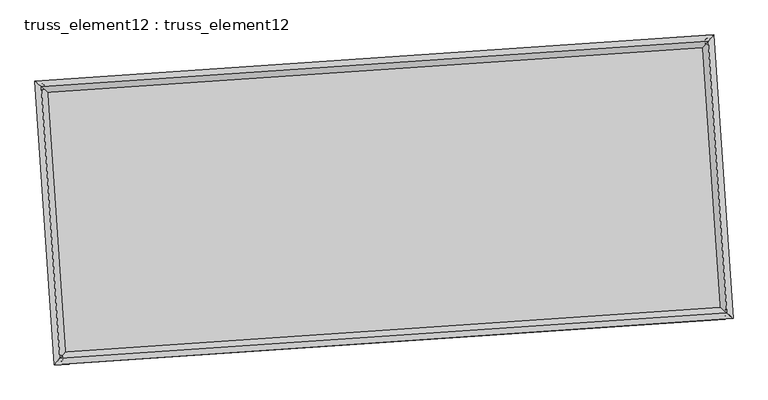
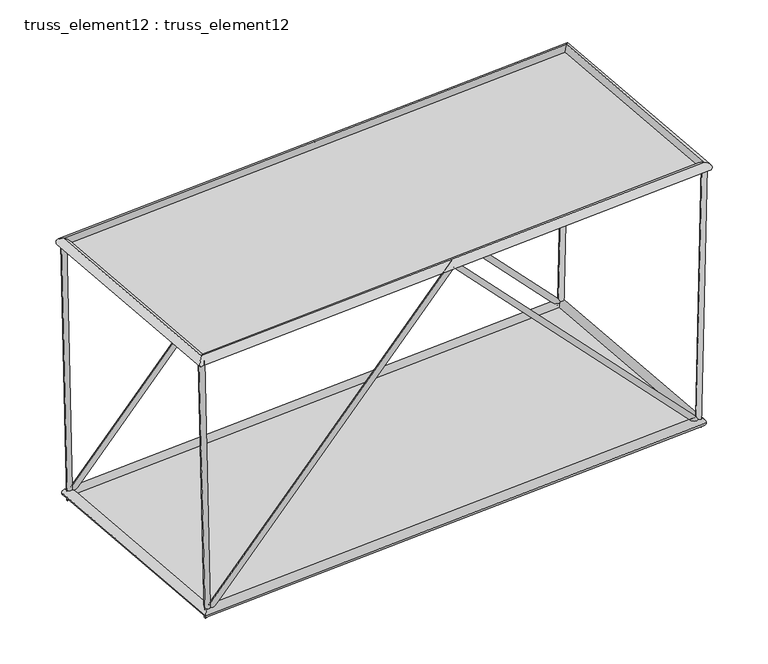
"""IFC4 building model written with IfcOpenShell, lengths in millimetres: plate geometry, truss_element12 : truss_element12."""

from ifc_helpers import new_model, si_unit, frame, origin, origin_with_axes, place, context, project, spatial, polyline, circle_curve, ellipse_curve, outline, extrude, source, transform, mapped, element, save
from ifc_brep_helpers import plane_surface, cylinder_surface, advanced_brep


def truss_element12_truss_element12_67497611(model_context):
    return source(origin(), model_context, "Body", "SolidModel", [
        advanced_brep(
        [(-3780.0029649, 2268.3783734, 4999.8207113), (-3879.0798521, 2255.0189396, 4997.5194202), (-3667.7199382, 2276.0345262, 121.2833616), (-3761.2669446, 2263.0521539, -121.2833616), (1063.4080842, 2598.6321613, 5070.7911986), (1063.8609339, 2592.0592819, 4926.563185), (5795.1440194, 2921.2712477, 121.2875843), (5889.6169576, 2921.1092408, -121.2875843), (5906.8236398, 2928.8862565, 4999.8287822), (6006.7972134, 2929.099317, 4997.5398535)],
        [
            (0, 1, circle_curve(frame((-3829.5414085, 2261.6986565, 4998.6700657), z_axis=(-0.023009593417978043, -0.0015689367075187464, 0.9997340131496714), x_axis=(-0.13359490987077044, 0.9910348587124408, -0.0015194977569957108)), 50.0)),
            (1, 0, circle_curve(frame((-3829.5414085, 2261.6986565, 4998.6700657), z_axis=(-0.023009593417978043, -0.0015689367075187464, 0.9997340131496714), x_axis=(-0.13359490987077044, 0.9910348587124408, -0.0015194977569957108)), 50.0)),
            (0, 2),
            (2, 3, ellipse_curve(frame((-3714.4934414, 2269.54334, 0.0), z_axis=(-0.9299983802713419, -0.06341305429589184, 0.36205220236527585), x_axis=(0.36121347081217686, 0.024629773473731183, 0.9321578207376976)), 130.3936428, 50.0)),
            (3, 1),
            (3, 2, ellipse_curve(frame((-3714.4934414, 2269.54334, 0.0), z_axis=(-0.9299983802713419, -0.06341305429589184, 0.36205220236527585), x_axis=(0.36121347081217686, 0.024629773473731183, 0.9321578207376976)), 130.3936428, 50.0)),
            (2, 4),
            (4, 5, ellipse_curve(frame((1063.6345091, 2595.3457216, 4998.6771918), z_axis=(-0.9976833955542868, -0.06802823819320505, -3.230475386094174e-05), x_axis=(3.22299165412689e-05, 2.1976354916597875e-06, -0.9999999994782015)), 72.2710337, 50.0)),
            (5, 3),
            (5, 4, ellipse_curve(frame((1063.6345091, 2595.3457216, 4998.6771918), z_axis=(-0.9976833955542868, -0.06802823819320505, -3.230475386094174e-05), x_axis=(3.22299165412689e-05, 2.1976354916597875e-06, -0.9999999994782015)), 72.2710337, 50.0)),
            (4, 6),
            (6, 7, ellipse_curve(frame((5842.3804885, 2921.1902443, 0.0), z_axis=(-0.9299643254301767, -0.0634107322257276, -0.36214007299081596), x_axis=(-0.3613011378762809, -0.02463575115757878, 0.9321236868217686)), 130.4029578, 50.0)),
            (7, 5),
            (7, 6, ellipse_curve(frame((5842.3804885, 2921.1902443, 0.0), z_axis=(-0.9299643254301767, -0.0634107322257276, -0.36214007299081596), x_axis=(-0.3613011378762809, -0.02463575115757878, 0.9321236868217686)), 130.4029578, 50.0)),
            (8, 9, circle_curve(frame((5956.8104266, 2928.9927867, 4998.6843179), z_axis=(0.02288598762129972, 0.001560508498112905, 0.9997368635715226), x_axis=(-0.002165762489590564, 0.9999965126634012, -0.0015113351298953748)), 50.0)),
            (9, 8, circle_curve(frame((5956.8104266, 2928.9927867, 4998.6843179), z_axis=(0.02288598762129972, 0.001560508498112905, 0.9997368635715226), x_axis=(-0.002165762489590564, 0.9999965126634012, -0.0015113351298953748)), 50.0)),
            (6, 8),
            (9, 7),
        ],
        [
            plane_surface(frame((-3829.5414085, 2311.6985949, 4998.7485334), z_axis=(-0.023009593417979597, -0.0015689367075153488, 0.9997340131496715), x_axis=(0.9997352442575682, -3.611015610971435e-05, 0.023009565083185635))),
            cylinder_surface(frame((-3829.5414085, 2261.6986565, 4998.6700657), z_axis=(-0.023009593417978046, -0.0015689367075187469, 0.9997340131496716), x_axis=(-0.13359490987077044, 0.9910348587124408, -0.0015194977569957108)), 50.0),
            cylinder_surface(frame((-3714.4934414, 2269.54334, 0.0), z_axis=(-0.6902141194664027, -0.04706307705691265, -0.7220730822203205), x_axis=(-0.02041714812690732, 0.9987520200568047, -0.04558006685839855)), 50.0),
            cylinder_surface(frame((1063.6345091, 2595.3457216, 4998.6771918), z_axis=(-0.6902606627361209, -0.04706625066554735, 0.722028382771328), x_axis=(-0.11534077341471446, 0.9922795388869102, -0.045583140463075246)), 50.0),
            plane_surface(frame((5956.8104266, 2878.9928477, 4998.7623637), z_axis=(0.022885987621301448, 0.0015605084981140682, 0.9997368635715226), x_axis=(0.9997380814846446, -3.572313472055558e-05, -0.02288595974085441))),
            cylinder_surface(frame((5842.3804885, 2921.1902443, 0.0), z_axis=(-0.02288598762129972, -0.001560508498112905, -0.9997368635715226), x_axis=(-0.002165762489590564, 0.9999965126634012, -0.0015113351298953748)), 50.0),
        ],
        [
            (0, [[1, 2]]),
            (1, [[-1, 3, 4, 5]]),
            (1, [[-2, -5, 6, -3]]),
            (2, [[-4, 7, 8, 9]]),
            (2, [[-6, -9, 10, -7]]),
            (3, [[-8, 11, 12, 13]]),
            (3, [[-10, -13, 14, -11]]),
            (4, [[15, 16]]),
            (5, [[-12, 17, -16, 18]]),
            (5, [[-14, -18, -15, -17]]),
        ],
    ),
        advanced_brep(
        [(-3507.890012, -1722.3552109, 4999.8207113), (-3606.9668992, -1735.7146447, 4997.5194202), (-3395.6069853, -1714.6990581, 121.2833616), (-3489.1539917, -1727.6814304, -121.2833616), (1335.5210371, -1392.101423, 5070.7911986), (1335.9738868, -1398.6743024, 4926.563185), (6067.2569723, -1069.4623366, 121.2875843), (6161.7299105, -1069.6243435, -121.2875843), (6178.9365927, -1061.8473278, 4999.8287822), (6278.9101663, -1061.6342673, 4997.5398535)],
        [
            (0, 1, circle_curve(frame((-3557.4284556, -1729.0349278, 4998.6700657), z_axis=(-0.02300959341797794, -0.0015689367075187003, 0.9997340131496715), x_axis=(-0.13359490987077055, 0.9910348587124407, -0.0015194977569957455)), 50.0)),
            (1, 0, circle_curve(frame((-3557.4284556, -1729.0349278, 4998.6700657), z_axis=(-0.02300959341797794, -0.0015689367075187003, 0.9997340131496715), x_axis=(-0.13359490987077055, 0.9910348587124407, -0.0015194977569957455)), 50.0)),
            (0, 2),
            (2, 3, ellipse_curve(frame((-3442.3804885, -1721.1902443, 0.0), z_axis=(-0.9299983802713419, -0.0634130542958918, 0.3620522023652762), x_axis=(0.3612134708121772, 0.02462977347373123, 0.9321578207376975)), 130.3936428, 50.0)),
            (3, 1),
            (3, 2, ellipse_curve(frame((-3442.3804885, -1721.1902443, 0.0), z_axis=(-0.9299983802713419, -0.0634130542958918, 0.3620522023652762), x_axis=(0.3612134708121772, 0.02462977347373123, 0.9321578207376975)), 130.3936428, 50.0)),
            (2, 4),
            (4, 5, ellipse_curve(frame((1335.747462, -1395.3878627, 4998.6771918), z_axis=(-0.9976833955542868, -0.06802823819320494, -3.230475386070103e-05), x_axis=(3.222991654111514e-05, 2.1976354915444677e-06, -0.9999999994782015)), 72.2710337, 50.0)),
            (5, 3),
            (5, 4, ellipse_curve(frame((1335.747462, -1395.3878627, 4998.6771918), z_axis=(-0.9976833955542868, -0.06802823819320494, -3.230475386070103e-05), x_axis=(3.222991654111514e-05, 2.1976354915444677e-06, -0.9999999994782015)), 72.2710337, 50.0)),
            (4, 6),
            (6, 7, ellipse_curve(frame((6114.4934414, -1069.54334, 0.0), z_axis=(-0.9299643254301767, -0.0634107322257272, -0.36214007299081574), x_axis=(-0.3613011378762808, -0.02463575115757876, 0.9321236868217685)), 130.4029578, 50.0)),
            (7, 5),
            (7, 6, ellipse_curve(frame((6114.4934414, -1069.54334, 0.0), z_axis=(-0.9299643254301767, -0.0634107322257272, -0.36214007299081574), x_axis=(-0.3613011378762808, -0.02463575115757876, 0.9321236868217685)), 130.4029578, 50.0)),
            (8, 9, circle_curve(frame((6228.9233795, -1061.7407976, 4998.6843179), z_axis=(0.02288598762129982, 0.0015605084981127825, 0.9997368635715226), x_axis=(-0.002165762489590051, 0.9999965126634012, -0.001511335129895264)), 50.0)),
            (9, 8, circle_curve(frame((6228.9233795, -1061.7407976, 4998.6843179), z_axis=(0.02288598762129982, 0.0015605084981127825, 0.9997368635715226), x_axis=(-0.002165762489590051, 0.9999965126634012, -0.001511335129895264)), 50.0)),
            (6, 8),
            (9, 7),
        ],
        [
            plane_surface(frame((-3557.4284556, -1679.0349894, 4998.7485334), z_axis=(-0.023009593417979597, -0.0015689367075153446, 0.9997340131496715), x_axis=(0.9997352442575682, -3.611015610971435e-05, 0.023009565083185635))),
            cylinder_surface(frame((-3557.4284556, -1729.0349278, 4998.6700657), z_axis=(-0.023009593417977935, -0.0015689367075186998, 0.9997340131496713), x_axis=(-0.13359490987077055, 0.9910348587124407, -0.0015194977569957455)), 50.0),
            cylinder_surface(frame((-3442.3804885, -1721.1902443, 0.0), z_axis=(-0.6902141194664028, -0.04706307705691266, -0.7220730822203204), x_axis=(-0.0204171481269073, 0.9987520200568046, -0.04558006685839858)), 50.0),
            cylinder_surface(frame((1335.747462, -1395.3878627, 4998.6771918), z_axis=(-0.6902606627361206, -0.04706625066554716, 0.7220283827713282), x_axis=(-0.11534077341471438, 0.9922795388869101, -0.04558314046307537)), 50.0),
            plane_surface(frame((6228.9233795, -1111.7407366, 4998.7623637), z_axis=(0.022885987621301448, 0.001560508498114064, 0.9997368635715226), x_axis=(0.9997380814846446, -3.572313472099967e-05, -0.02288595974085441))),
            cylinder_surface(frame((6114.4934414, -1069.54334, 0.0), z_axis=(-0.02288598762129982, -0.0015605084981127825, -0.9997368635715226), x_axis=(-0.002165762489590051, 0.9999965126634012, -0.001511335129895264)), 50.0),
        ],
        [
            (0, [[1, 2]]),
            (1, [[-1, 3, 4, 5]]),
            (1, [[-2, -5, 6, -3]]),
            (2, [[-4, 7, 8, 9]]),
            (2, [[-6, -9, 10, -7]]),
            (3, [[-8, 11, 12, 13]]),
            (3, [[-10, -13, 14, -11]]),
            (4, [[15, 16]]),
            (5, [[-12, 17, -16, 18]]),
            (5, [[-14, -18, -15, -17]]),
        ],
    ),
        advanced_brep(
        [(-3557.4247553, -1729.0308266, 4908.6700658), (-3557.4321559, -1729.039029, 5088.6700657), (-3829.5456313, 2261.7022175, 5088.6700657), (-3829.5371857, 2261.6950955, 4908.6700658), (5956.813866, 2928.9968702, 5088.6843178), (5956.8069872, 2928.9887033, 4908.6843179), (6228.9273414, -1061.7443763, 5088.6843178), (6228.9194177, -1061.7372188, 4908.6843179)],
        [
            (0, 1, ellipse_curve(frame((-3557.4284556, -1729.0349278, 4998.6700657), z_axis=(-0.7535719234047118, 0.6573654662781334, -1.0273917259752128e-06), x_axis=(-0.657365466277338, -0.7535719234054056, -1.0273917259753225e-06)), 127.2792206, 90.0)),
            (1, 2),
            (2, 3, ellipse_curve(frame((-3829.5414085, 2261.6986565, 4998.6700657), z_axis=(-0.657365466277338, -0.7535719234054056, -1.027391725975426e-06), x_axis=(0.7535719234047117, -0.6573654662781334, 1.0273917259753161e-06)), 127.2792206, 90.0)),
            (3, 0),
            (1, 0, ellipse_curve(frame((-3557.4284556, -1729.0349278, 4998.6700657), z_axis=(-0.7535719234047118, 0.6573654662781334, -1.0273917259752128e-06), x_axis=(-0.657365466277338, -0.7535719234054056, -1.0273917259753225e-06)), 127.2792206, 90.0)),
            (3, 2, ellipse_curve(frame((-3829.5414085, 2261.6986565, 4998.6700657), z_axis=(-0.657365466277338, -0.7535719234054056, -1.027391725975426e-06), x_axis=(0.7535719234047117, -0.6573654662781334, 1.0273917259753161e-06)), 127.2792206, 90.0)),
            (2, 4),
            (4, 5, ellipse_curve(frame((5956.8104266, 2928.9927867, 4998.6843179), z_axis=(-0.7535719234047119, 0.6573654662781332, -1.027391725975419e-06), x_axis=(-0.6573654662773378, -0.7535719234054058, -1.0273917259753231e-06)), 127.2792206, 90.0)),
            (5, 3),
            (5, 4, ellipse_curve(frame((5956.8104266, 2928.9927867, 4998.6843179), z_axis=(-0.7535719234047119, 0.6573654662781332, -1.027391725975419e-06), x_axis=(-0.6573654662773378, -0.7535719234054058, -1.0273917259753231e-06)), 127.2792206, 90.0)),
            (4, 6),
            (6, 7, ellipse_curve(frame((6228.9233795, -1061.7407976, 4998.6843179), z_axis=(0.6573654662773379, 0.7535719234054057, 1.0273917259752202e-06), x_axis=(-0.7535719234047118, 0.6573654662781332, -1.0273917259753155e-06)), 127.2792206, 90.0)),
            (7, 5),
            (7, 6, ellipse_curve(frame((6228.9233795, -1061.7407976, 4998.6843179), z_axis=(0.6573654662773379, 0.7535719234054057, 1.0273917259752202e-06), x_axis=(-0.7535719234047118, 0.6573654662781332, -1.0273917259753155e-06)), 127.2792206, 90.0)),
            (6, 1),
            (0, 7),
        ],
        [
            cylinder_surface(frame((-3557.4284556, -1729.0349278, 4998.6700657), z_axis=(0.06802823822869923, -0.9976833960748768, 0.0), x_axis=(-0.9976833951038621, -0.06802823816248943, -4.4119596619709036e-05)), 90.0),
            cylinder_surface(frame((-3829.5414085, 2261.6986565, 4998.6700657), z_axis=(-0.9976833960738238, -0.0680282382286269, -1.4529513127442725e-06), x_axis=(-0.06802823810492901, 0.9976833951709815, -4.266664530828733e-05)), 90.0),
            cylinder_surface(frame((5956.8104266, 2928.9927867, 4998.6843179), z_axis=(-0.06802823822869945, 0.9976833960748768, 0.0), x_axis=(0.9976833952275599, 0.06802823817092414, -4.1213693996865644e-05)), 90.0),
            cylinder_surface(frame((6228.9233795, -1061.7407976, 4998.6843179), z_axis=(0.9976833960738237, 0.06802823822862669, 1.4529513127441262e-06), x_axis=(0.06802823822862669, -0.9976833951625469, -4.266664530828735e-05)), 90.0),
        ],
        [
            (0, [[1, 2, 3, 4]]),
            (0, [[5, -4, 6, -2]]),
            (1, [[-3, 7, 8, 9]]),
            (1, [[-6, -9, 10, -7]]),
            (2, [[-8, 11, 12, 13]]),
            (2, [[-10, -13, 14, -11]]),
            (3, [[-12, 15, -1, 16]]),
            (3, [[-14, -16, -5, -15]]),
        ],
    ),
        advanced_brep(
        [(-3358.7115243, -1625.2761972, 0.0), (-3526.0494527, -1817.1042913, 0.0), (-3810.4074885, 2353.2123043, 0.0), (-3618.5793943, 2185.8743758, 0.0), (5926.0494527, 3017.1042913, 0.0), (5758.7115243, 2825.2761972, 0.0), (6210.4074885, -1153.2123043, 0.0), (6018.5793943, -985.8743758, 0.0)],
        [
            (0, 1, ellipse_curve(frame((-3442.3804885, -1721.1902443, 0.0), z_axis=(-0.7535719234054586, 0.6573654662780799, 0.0), x_axis=(-0.6573654662780799, -0.7535719234054586, 0.0)), 127.2792206, 90.0)),
            (1, 2),
            (2, 3, ellipse_curve(frame((-3714.4934414, 2269.54334, 0.0), z_axis=(-0.6573654662780799, -0.7535719234054585, 0.0), x_axis=(0.7535719234054584, -0.6573654662780802, 0.0)), 127.2792206, 90.0)),
            (3, 0),
            (1, 0, ellipse_curve(frame((-3442.3804885, -1721.1902443, 0.0), z_axis=(-0.7535719234054586, 0.6573654662780799, 0.0), x_axis=(-0.6573654662780799, -0.7535719234054586, 0.0)), 127.2792206, 90.0)),
            (3, 2, ellipse_curve(frame((-3714.4934414, 2269.54334, 0.0), z_axis=(-0.6573654662780799, -0.7535719234054585, 0.0), x_axis=(0.7535719234054584, -0.6573654662780802, 0.0)), 127.2792206, 90.0)),
            (2, 4),
            (4, 5, ellipse_curve(frame((5842.3804885, 2921.1902443, 0.0), z_axis=(-0.753571923405459, 0.6573654662780798, 0.0), x_axis=(-0.6573654662780796, -0.753571923405459, 0.0)), 127.2792206, 90.0)),
            (5, 3),
            (5, 4, ellipse_curve(frame((5842.3804885, 2921.1902443, 0.0), z_axis=(-0.753571923405459, 0.6573654662780798, 0.0), x_axis=(-0.6573654662780796, -0.753571923405459, 0.0)), 127.2792206, 90.0)),
            (4, 6),
            (6, 7, ellipse_curve(frame((6114.4934414, -1069.54334, 0.0), z_axis=(0.6573654662780798, 0.7535719234054588, 0.0), x_axis=(-0.7535719234054588, 0.65736546627808, 0.0)), 127.2792206, 90.0)),
            (7, 5),
            (7, 6, ellipse_curve(frame((6114.4934414, -1069.54334, 0.0), z_axis=(0.6573654662780798, 0.7535719234054588, 0.0), x_axis=(-0.7535719234054588, 0.65736546627808, 0.0)), 127.2792206, 90.0)),
            (6, 1),
            (0, 7),
        ],
        [
            cylinder_surface(frame((-3442.3804885, -1721.1902443, 0.0), z_axis=(0.06802823822870264, -0.9976833960748764, 0.0), x_axis=(-0.9976833960748764, -0.06802823822870264, 0.0)), 90.0),
            cylinder_surface(frame((-3714.4934414, 2269.54334, 0.0), z_axis=(-0.9976833960748767, -0.06802823822870221, 0.0), x_axis=(-0.06802823822870221, 0.9976833960748767, 0.0)), 90.0),
            cylinder_surface(frame((5842.3804885, 2921.1902443, 0.0), z_axis=(-0.06802823822870314, 0.9976833960748764, 0.0), x_axis=(0.9976833960748764, 0.06802823822870314, 0.0)), 90.0),
            cylinder_surface(frame((6114.4934414, -1069.54334, 0.0), z_axis=(0.9976833960748765, 0.06802823822870205, 0.0), x_axis=(0.06802823822870205, -0.9976833960748765, 0.0)), 90.0),
        ],
        [
            (0, [[1, 2, 3, 4]]),
            (0, [[5, -4, 6, -2]]),
            (1, [[-3, 7, 8, 9]]),
            (1, [[-6, -9, 10, -7]]),
            (2, [[-8, 11, 12, 13]]),
            (2, [[-10, -13, 14, -11]]),
            (3, [[-12, 15, -1, 16]]),
            (3, [[-14, -16, -5, -15]]),
        ],
    ),
        extrude(outline(polyline([(-3442.3804885, -1721.1902443), (-3714.4934414, 2269.54334), (5842.3804885, 2921.1902443), (6114.4934414, -1069.54334), (-3442.3804885, -1721.1902443)])), origin_with_axes(), (0.0, 0.0, 1.0), 20.0),
        extrude(outline(polyline([(-2000.0, 4904.5377891), (2000.0, 4904.537789), (1999.9999999, -4904.5377891), (-2000.0000001, -4904.537789), (-2000.0, 4904.5377891)])), frame((1199.6909855, 599.9789295, 4998.6771918), z_axis=(-1.4495854000300826e-06, -9.884171803806847e-08, 0.9999999999989445), x_axis=(-0.06802823822870253, 0.9976833960748765, 0.0)), (0.0, 0.0, 1.0), 20.0),
    ])


if __name__ == "__main__":
    model = new_model("IFC4")
    model_context = context("Model", 3, world=origin())
    ifc_project = project(units=[si_unit("LENGTHUNIT", "METRE", prefix="MILLI")], contexts=[model_context])
    site = spatial("IfcSite", under=ifc_project)
    building = spatial("IfcBuilding", under=site)
    placement = place(None, origin())
    truss_element12_truss_element12_shape = truss_element12_truss_element12_67497611(model_context)
    element("IfcPlate", 1, ObjectType="truss_element12 : truss_element12", at=placement, inside=building, context=model_context, shape_type="MappedRepresentation", body=[
        mapped(truss_element12_truss_element12_shape, transform((0.0, 0.0, 0.0), x_axis=(1.0, 0.0, 0.0), y_axis=(0.0, 1.0, 0.0), z_axis=(0.0, 0.0, 1.0))),
    ])
    save(model, "model.ifc")

# Revit data of these elements
# Type "truss_element12 : truss_element12"
#   steellbar1 = 90 mm
#   steelbar2 = 50 mm
#   offset1 = 5000 mm
#   M = Default Roof
# Element 1 (IfcPlate, "truss_element12 : truss_element12")
#   Materials on its faces: "Default Roof"
# Materials
#   "Default Roof": class "Miscellaneous", colour RGB 0 127 0, transparency 0, Comments = "Rendering appearance not upgraded Rendering appearance not upgraded ", Cost = 0
